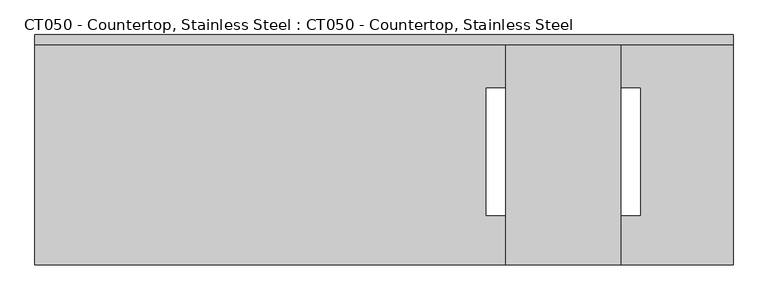
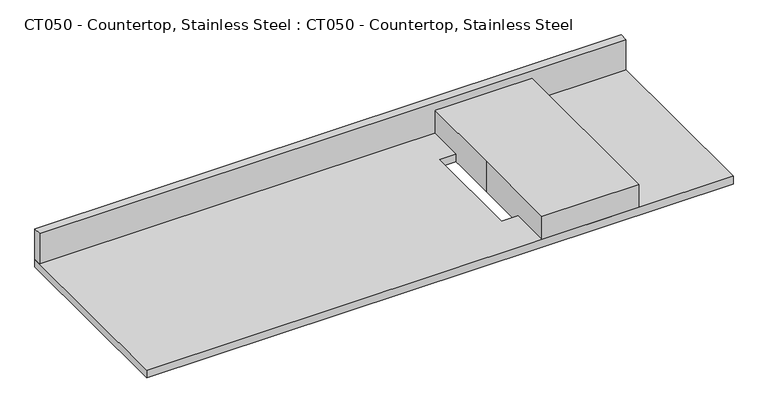
"""IFC4 building model written with IfcOpenShell, lengths in millimetres: proxy geometry, CT050 - Countertop, Stainless Steel : CT050 - Countertop, Stainless Steel."""

from ifc_helpers import new_model, si_unit, frame, origin, origin_with_axes, place, context, project, spatial, polyline, outline, extrude, source, transform, mapped, element, save


def ct050_countertop_stainless_steel_ct050_countertop_stainless_ed4b3b38(model_context):
    return source(origin(), model_context, "Body", "SweptSolid", [
        extrude(outline(polyline([(449.2625, 304.8), (449.2625, -304.8), (-1397.0, -304.8), (-1397.0, 304.8), (449.2625, 304.8)]), holes=[polyline([(203.1999999, 164.3131965), (-203.2000001, 164.3131965), (-203.2000001, -172.9014465), (203.1999999, -172.9014465), (203.1999999, 164.3131965)])]), origin_with_axes(), (0.0, 0.0, 1.0), 25.4),
        extrude(outline(polyline([(-1397.0, 279.4), (-1397.0, 304.8), (449.2625, 304.8), (449.2625, 279.4), (-1397.0, 279.4)])), frame((0.0, 0.0, 25.4), z_axis=(0.0, 0.0, 1.0), x_axis=(1.0, 0.0, 0.0)), (0.0, 0.0, 1.0), 101.6),
        extrude(outline(polyline([(-152.4, 304.8), (152.4, 304.8), (152.4, -304.8), (-152.4, -304.8), (-152.4, 0.0), (-152.4, 304.8)])), origin_with_axes(), (0.0, 0.0, 1.0), 101.6),
    ])


if __name__ == "__main__":
    model = new_model("IFC4")
    model_context = context("Model", 3, world=origin())
    ifc_project = project(units=[si_unit("LENGTHUNIT", "METRE", prefix="MILLI")], contexts=[model_context])
    site = spatial("IfcSite", under=ifc_project)
    building = spatial("IfcBuilding", under=site)
    placement = place(None, origin())
    ct050_countertop_stainless_steel_ct050_countertop_stainless_shape = ct050_countertop_stainless_steel_ct050_countertop_stainless_ed4b3b38(model_context)
    element("IfcBuildingElementProxy", 1, Name="CT050 - Countertop, Stainless Steel : CT050 - Countertop, Stainless Steel", ObjectType="CT050 - Countertop, Stainless Steel : CT050 - Countertop, Stainless Steel", at=placement, inside=building, context=model_context, shape_type="MappedRepresentation", body=[
        mapped(ct050_countertop_stainless_steel_ct050_countertop_stainless_shape, transform((0.0, 0.0, 0.0), x_axis=(1.0, 0.0, 0.0), y_axis=(0.0, 1.0, 0.0), z_axis=(0.0, 0.0, 1.0))),
    ])
    save(model, "model.ifc")

# Revit data of these elements
# Type "CT050 - Countertop, Stainless Steel : CT050 - Countertop, Stainless Steel"
#   Watts2 = "0"
#   Watts1 = "0"
#   Unit_Issue = "LF"
#   UTIL_6_Misc = "-"
#   UTIL_5_NonMedGas = "-"
#   UTIL_4_MiscGas = "-"
#   UTIL_3_MedGas = "-"
#   UTIL_2_Elec = "-"
#   UTIL_1_WaterDrain = "-"
#   Nomenclature = "Countertop, Stainless Steel"
#   NSN = "6530"
#   Location [instance default] = ""
#   JSN = "CT050"
#   Fund_Source_VA = "-"
#   Fund_Source_Navy = "-"
#   Fund_Source_Army = "-"
#   Fund_Source_AF = "-"
#   ELEC_Volts2 = "0"
#   ELEC_Volts1 = "0"
#   ELEC_Phase2 = "0"
#   ELEC_Phase1 = "0"
#   ELEC_HertzSwitch = "0"
#   ELEC_HertzDependent = "0"
#   ELEC_Hertz = "0"
#   ELEC_Amps2 = "0"
#   ELEC_Amps1 = "0"
#   DetailDescription = "Stainless steel countertop (composition of heavy-gauge Type No. 304 stainless steel) having a smooth satin finish and integral 4\" backsplash/curb. Also referred to as a corrosion-resistant steel work surface or work top. Available in various depths. Used in areas where excellent ease of cleaning, abrasion resistance, bacteria resistance, impact resistance, load capacity and moisture resistance, are of concern. Pricing based upon a 24\" depth."
#   CAT_VA = "A"
#   CAT_Navy = "A"
#   CAT_IHS = "-"
#   CAT_Army = "A"
#   CAT_AF = "A"
#   BTUperhour = "0"
#   Weight_IP = 0
#   OpeningLength2 [instance default] = 0' - 3"
#   OpeningLength [instance default] = 0' - 3"
#   OpeningDepth2 [instance default] = 0' - 3"
#   OpeningDepth [instance default] = 0' - 3"
#   DIM_Width_IP = 1' - 0"
#   DIM_Height_IP = 0' - 4"
#   DIM_Depth_IP = 2' - 0"
#   CustomLength2 [instance default] = 1' - 6"
#   CustomLength [instance default] = 1' - 6"
#   Assembly Code = ""
# Element 1 (IfcBuildingElementProxy, "CT050 - Countertop, Stainless Steel : CT050 - Countertop, Stainless Steel")
#   Location = "ORSR1"
#   OpeningLength2 = 0' - 8"
#   OpeningLength = 0' - 8"
#   OpeningDepth2 = 0' - 6.80714"
#   OpeningDepth = 0' - 6.46902"
#   CustomLength2 = 1' - 5 11/16"
#   CustomLength = 4' - 7"
#   Materials on its faces: "CounterTopFinish - Stainless", "EquipSpace"
# Materials
#   "CounterTopFinish - Stainless": class "Unassigned", colour RGB 187 187 187, transparency 0
#   "EquipSpace": class "Unassigned", colour RGB 221 217 195, transparency 0.5
